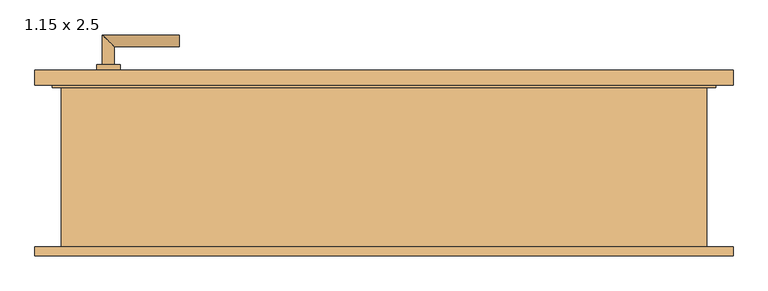
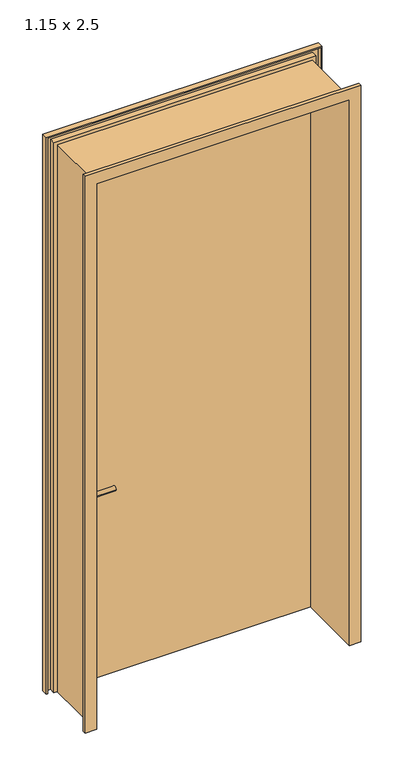
"""IFC4 building model written with IfcOpenShell, lengths in millimetres: door geometry, Drehflügel 1-flg - Stahlzarge : 1.15 x 2.5."""

from ifc_helpers import new_model, si_unit, point, frame, frame_2d, origin, place, context, project, spatial, polyline, circle_curve, ellipse_curve, trimmed, segment, composite_curve, outline, extrude, faceted_brep, source, transform, mapped, element, save
from ifc_brep_helpers import plane_surface, cylinder_surface, advanced_brep


def door_1_15_x_2_5_18a13e10(model_context):
    return source(origin(), model_context, "Body", "SolidModel", [
        advanced_brep(
        [(-477.5, 126.9346141, 901.0), (-457.5, 126.9346141, 901.0), (-477.5, 56.9346141, 901.0), (-457.5, 76.9346141, 901.0), (-347.5, 56.9346141, 901.0), (-347.5, 76.9346141, 901.0)],
        [
            (0, 1, circle_curve(frame((-467.5, 126.9346141, 901.0), z_axis=(0.0, 1.0, 0.0), x_axis=(1.0, 0.0, 0.0)), 10.0)),
            (1, 0, circle_curve(frame((-467.5, 126.9346141, 901.0), z_axis=(0.0, 1.0, 0.0), x_axis=(1.0, 0.0, 0.0)), 10.0)),
            (0, 2),
            (2, 3, ellipse_curve(frame((-467.5, 66.9346141, 901.0), z_axis=(-0.7071067811865385, 0.7071067811865565, 0.0), x_axis=(0.7071067811865563, 0.7071067811865386, 0.0)), 14.1421356, 10.0)),
            (3, 1),
            (3, 2, ellipse_curve(frame((-467.5, 66.9346141, 901.0), z_axis=(-0.7071067811865385, 0.7071067811865565, 0.0), x_axis=(0.7071067811865563, 0.7071067811865386, 0.0)), 14.1421356, 10.0)),
            (4, 5, circle_curve(frame((-347.5, 66.9346141, 901.0), z_axis=(1.0, 0.0, 0.0), x_axis=(0.0, 1.0, 0.0)), 10.0)),
            (5, 4, circle_curve(frame((-347.5, 66.9346141, 901.0), z_axis=(1.0, 0.0, 0.0), x_axis=(0.0, 1.0, 0.0)), 10.0)),
            (2, 4),
            (5, 3),
        ],
        [
            plane_surface(frame((-467.5, 126.9346141, -386.7526403), z_axis=(0.0, 1.0, 0.0), x_axis=(0.0, 0.0, 1.0))),
            cylinder_surface(frame((-467.5, 126.9346141, 901.0), z_axis=(0.0, 1.0, 0.0), x_axis=(1.0, 0.0, 0.0)), 10.0),
            plane_surface(frame((-347.5, 66.9346141, -386.7526403), z_axis=(1.0, 0.0, 0.0), x_axis=(0.0, 0.0, 1.0))),
            cylinder_surface(frame((-467.5, 66.9346141, 901.0), z_axis=(-1.0, 0.0, 0.0), x_axis=(0.0, 1.0, 0.0)), 10.0),
        ],
        [
            (0, [[1, 2]]),
            (1, [[-1, 3, 4, 5]]),
            (1, [[-2, -5, 6, -3]]),
            (2, [[7, 8]]),
            (3, [[-4, 9, -8, 10]]),
            (3, [[-6, -10, -7, -9]]),
        ],
    ),
        advanced_brep(
        [(-457.5, 186.9346141, 901.0), (-477.5, 186.9346141, 901.0), (-457.5, 216.9346141, 901.0), (-477.5, 236.9346141, 901.0), (-347.5, 216.9346141, 901.0), (-347.5, 236.9346141, 901.0)],
        [
            (0, 1, circle_curve(frame((-467.5, 186.9346141, 901.0), z_axis=(0.0, -1.0, 0.0), x_axis=(-1.0, 0.0, 0.0)), 10.0)),
            (1, 0, circle_curve(frame((-467.5, 186.9346141, 901.0), z_axis=(0.0, -1.0, 0.0), x_axis=(-1.0, 0.0, 0.0)), 10.0)),
            (0, 2),
            (2, 3, ellipse_curve(frame((-467.5, 226.9346141, 901.0), z_axis=(-0.7071067811865475, -0.7071067811865475, 0.0), x_axis=(0.7071067811865474, -0.7071067811865476, 0.0)), 14.1421356, 10.0)),
            (3, 1),
            (3, 2, ellipse_curve(frame((-467.5, 226.9346141, 901.0), z_axis=(-0.7071067811865475, -0.7071067811865475, 0.0), x_axis=(0.7071067811865474, -0.7071067811865476, 0.0)), 14.1421356, 10.0)),
            (4, 5, circle_curve(frame((-347.5, 226.9346141, 901.0), z_axis=(1.0, 0.0, 0.0), x_axis=(0.0, 1.0, 0.0)), 10.0)),
            (5, 4, circle_curve(frame((-347.5, 226.9346141, 901.0), z_axis=(1.0, 0.0, 0.0), x_axis=(0.0, 1.0, 0.0)), 10.0)),
            (2, 4),
            (5, 3),
        ],
        [
            plane_surface(frame((-467.5, 186.9346141, -386.7526403), z_axis=(0.0, -1.0, 0.0), x_axis=(0.0, 0.0, 1.0))),
            cylinder_surface(frame((-467.5, 186.9346141, 901.0), z_axis=(0.0, -1.0, 0.0), x_axis=(-1.0, 0.0, 0.0)), 10.0),
            plane_surface(frame((-347.5, 226.9346141, -386.7526403), z_axis=(1.0, 0.0, 0.0), x_axis=(0.0, 0.0, 1.0))),
            cylinder_surface(frame((-467.5, 226.9346141, 901.0), z_axis=(-1.0, 0.0, 0.0), x_axis=(0.0, 1.0, 0.0)), 10.0),
        ],
        [
            (0, [[1, 2]]),
            (1, [[-1, 3, 4, 5]]),
            (1, [[-2, -5, 6, -3]]),
            (2, [[7, 8]]),
            (3, [[-4, 9, -8, 10]]),
            (3, [[-6, -10, -7, -9]]),
        ],
    ),
        extrude(outline(composite_curve([segment(trimmed(circle_curve(frame_2d((901.0, -467.5)), 20.0), [point((901.0, -487.5))], [point((901.0, -447.5))], False, "CARTESIAN"), True, "CONTINUOUS"), segment(trimmed(circle_curve(frame_2d((901.0, -467.5)), 20.0), [point((901.0, -447.5))], [point((901.0, -487.5))], False, "CARTESIAN"), True, "CONTINUOUS")], self_intersect=False)), frame((0.0, 116.9346141, 0.0), z_axis=(0.0, 1.0, 0.0), x_axis=(0.0, 0.0, 1.0)), (0.0, 0.0, 1.0), 10.0),
        extrude(outline(composite_curve([segment(trimmed(circle_curve(frame_2d((901.0, -467.5)), 20.0), [point((901.0, -487.5))], [point((901.0, -447.5))], False, "CARTESIAN"), True, "CONTINUOUS"), segment(trimmed(circle_curve(frame_2d((901.0, -467.5)), 20.0), [point((901.0, -447.5))], [point((901.0, -487.5))], False, "CARTESIAN"), True, "CONTINUOUS")], self_intersect=False)), frame((0.0, 176.9346141, 0.0), z_axis=(0.0, 1.0, 0.0), x_axis=(0.0, 0.0, 1.0)), (0.0, 0.0, 1.0), 10.0),
        extrude(outline(polyline([(557.5, 151.9346141), (-557.5, 151.9346141), (-557.5, 176.9346141), (557.5, 176.9346141), (557.5, 151.9346141)])), frame((0.0, 0.0, 1.0), z_axis=(0.0, 0.0, 1.0), x_axis=(1.0, 0.0, 0.0)), (0.0, 0.0, 1.0), 2490.0),
        faceted_brep([(591.9603207, -138.0653859, 1.0), (542.5, -138.0653859, 1.0), (542.5, 151.9346141, 1.0), (557.5, 151.9346141, 1.0), (557.5, 176.9346141, 1.0), (591.9603207, 176.9346141, 1.0), (591.9603207, 151.9346141, 1.0), (586.9603207, 151.9346141, 1.0), (586.9603207, 171.9346141, 1.0), (562.5, 171.9346141, 1.0), (562.5, 146.9346141, 1.0), (547.5, 146.9346141, 1.0), (547.5, -133.0653859, 1.0), (586.9603207, -133.0653859, 1.0), (586.9603207, -123.0653859, 1.0), (591.9603207, -123.0653859, 1.0), (591.9603207, -138.0653859, 2525.4603207), (-591.9603207, -138.0653859, 2525.4603207), (-591.9603207, -138.0653859, 1.0), (-542.5, -138.0653859, 1.0), (-542.5, -138.0653859, 2476.0), (542.5, -138.0653859, 2476.0), (542.5, 151.9346141, 2476.0), (-542.5, 151.9346141, 2476.0), (-542.5, 151.9346141, 1.0), (-557.5, 151.9346141, 1.0), (-557.5, 151.9346141, 2491.0), (557.5, 151.9346141, 2491.0), (557.5, 176.9346141, 2491.0), (-557.5, 176.9346141, 2491.0), (-557.5, 176.9346141, 1.0), (-591.9603207, 176.9346141, 1.0), (-591.9603207, 176.9346141, 2525.4603207), (591.9603207, 176.9346141, 2525.4603207), (591.9603207, 151.9346141, 2525.4603207), (-591.9603207, 151.9346141, 2525.4603207), (-591.9603207, 151.9346141, 1.0), (-586.9603207, 151.9346141, 1.0), (-586.9603207, 151.9346141, 2520.4603207), (586.9603207, 151.9346141, 2520.4603207), (586.9603207, 171.9346141, 2520.4603207), (-586.9603207, 171.9346141, 2520.4603207), (-586.9603207, 171.9346141, 1.0), (-562.5, 171.9346141, 1.0), (-562.5, 171.9346141, 2496.0), (562.5, 171.9346141, 2496.0), (562.5, 146.9346141, 2496.0), (-562.5, 146.9346141, 2496.0), (-562.5, 146.9346141, 1.0), (-547.5, 146.9346141, 1.0), (-547.5, 146.9346141, 2481.0), (547.5, 146.9346141, 2481.0), (547.5, -133.0653859, 2481.0), (-547.5, -133.0653859, 2481.0), (-547.5, -133.0653859, 1.0), (-586.9603207, -133.0653859, 1.0), (-586.9603207, -133.0653859, 2520.4603207), (586.9603207, -133.0653859, 2520.4603207), (586.9603207, -123.0653859, 2520.4603207), (-586.9603207, -123.0653859, 2520.4603207), (-586.9603207, -123.0653859, 1.0), (-591.9603207, -123.0653859, 1.0), (-591.9603207, -123.0653859, 2525.4603207), (591.9603207, -123.0653859, 2525.4603207)], [[[0, 1, 2, 3, 4, 5, 6, 7, 8, 9, 10, 11, 12, 13, 14, 15]], [[1, 0, 16, 17, 18, 19, 20, 21]], [[2, 1, 21, 22]], [[3, 2, 22, 23, 24, 25, 26, 27]], [[4, 3, 27, 28]], [[5, 4, 28, 29, 30, 31, 32, 33]], [[6, 5, 33, 34]], [[7, 6, 34, 35, 36, 37, 38, 39]], [[8, 7, 39, 40]], [[9, 8, 40, 41, 42, 43, 44, 45]], [[10, 9, 45, 46]], [[11, 10, 46, 47, 48, 49, 50, 51]], [[12, 11, 51, 52]], [[13, 12, 52, 53, 54, 55, 56, 57]], [[14, 13, 57, 58]], [[15, 14, 58, 59, 60, 61, 62, 63]], [[0, 15, 63, 16]], [[17, 62, 61, 18]], [[18, 61, 60, 55, 54, 49, 48, 43, 42, 37, 36, 31, 30, 25, 24, 19]], [[23, 20, 19, 24]], [[29, 26, 25, 30]], [[35, 32, 31, 36]], [[41, 38, 37, 42]], [[47, 44, 43, 48]], [[53, 50, 49, 54]], [[59, 56, 55, 60]], [[22, 21, 20, 23]], [[28, 27, 26, 29]], [[34, 33, 32, 35]], [[40, 39, 38, 41]], [[46, 45, 44, 47]], [[52, 51, 50, 53]], [[58, 57, 56, 59]], [[16, 63, 62, 17]]]),
    ])


if __name__ == "__main__":
    model = new_model("IFC4")
    model_context = context("Model", 3, world=origin())
    ifc_project = project(units=[si_unit("LENGTHUNIT", "METRE", prefix="MILLI")], contexts=[model_context])
    site = spatial("IfcSite", under=ifc_project)
    building = spatial("IfcBuilding", under=site)
    placement = place(None, origin())
    door_1_15_x_2_5_shape = door_1_15_x_2_5_18a13e10(model_context)
    element("IfcDoor", 1, ObjectType="Drehflügel 1-flg - Stahlzarge : 1.15 x 2.5", at=placement, inside=building, context=model_context, shape_type="MappedRepresentation", body=[
        mapped(door_1_15_x_2_5_shape, transform((0.0, 0.0, 0.0), x_axis=(1.0, 0.0, 0.0), y_axis=(0.0, 1.0, 0.0), z_axis=(0.0, 0.0, 1.0))),
    ])
    save(model, "model.ifc")

# Revit data of these elements
# Type "Drehflügel 1-flg - Stahlzarge : 1.15 x 2.5"
#   Type Mark = "21"
#   Operation = "SingleSwingRight"
#   Keynote = "16.03"
#   Analytic Construction = "Metall"
#   Thermal Resistance (R) = 0.270117 (m²·K)/W
#   Heat Transfer Coefficient (U) = 3.7021 W/(m²·K)
#   Rough Width = 1.135 m
#   Rough Height [instance default] = 2.600 m
#   Höhe Türgriff [instance default] = 0.900 m
#   Height = 2.500 m
#   Fußbodenaufbau [instance default] = 0.100 m
#   Width = 1.135 m
#   Sichtbarkeit Sturzlinien [instance default] = yes
#   Türgriff auswählen [instance default] = element 221079
#   Türgriff [instance default] = none
#   Türflügel [instance default] = none
#   Rahmen/Pfosten [instance default] = Metall - Lackiert - Grau
#   Visual Light Transmittance = 0
#   Solar Heat Gain Coefficient = 0
#   Function = (empty or 0)
#   Wall Closure = (empty or 0)
# Element 1 (IfcDoor, "Drehflügel 1-flg - Stahlzarge : 1.15 x 2.5")
#   Rough Height = 2.501 m
#   Fußbodenaufbau = 0.001 m
#   Materials on its faces: "Metall - Lackiert - Grau", "Metall - Chrom", "Holz - Birke"
# Materials
#   "Metall - Lackiert - Grau": class "Farbe 1", colour RGB 98 98 98, transparency 0, Cost = 0
#   "Metall - Chrom": class "Metall", colour RGB 247 247 247, transparency 0, Cost = 0
#   "Holz - Birke": class "Holz", colour RGB 213 164 103, transparency 0, Cost = 0
